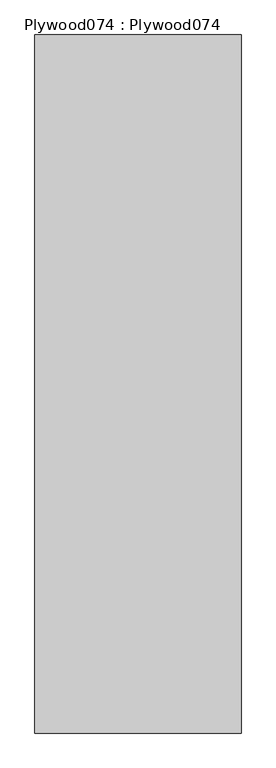
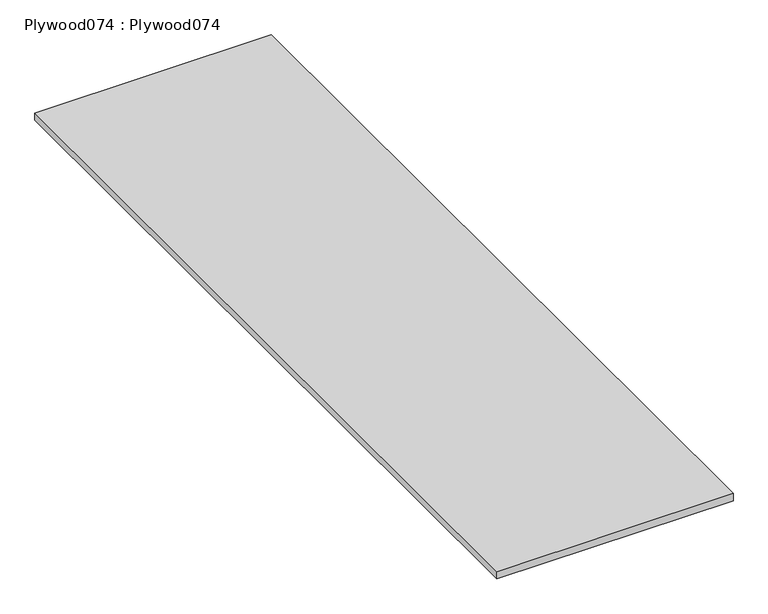
"""IFC4 building model written with IfcOpenShell, lengths in millimetres: proxy geometry, Plywood074 : Plywood074."""

from ifc_helpers import new_model, si_unit, frame, origin, place, context, project, spatial, polyline, outline, extrude, source, transform, mapped, element, save


def plywood074_plywood074_564b9597(model_context):
    return source(origin(), model_context, "Body", "SweptSolid", [
        extrude(outline(polyline([(-4404.2038825, -1052.8906574), (-4994.7538825, -1052.8906574), (-4994.7538825, 947.1093426), (-4404.2038825, 947.1093426), (-4404.2038825, -1052.8906574)])), frame((0.0, 0.0, 40112.696), z_axis=(0.0, 0.0, 1.0), x_axis=(1.0, 0.0, 0.0)), (0.0, 0.0, 1.0), 19.05),
    ])


if __name__ == "__main__":
    model = new_model("IFC4")
    model_context = context("Model", 3, world=origin())
    ifc_project = project(units=[si_unit("LENGTHUNIT", "METRE", prefix="MILLI")], contexts=[model_context])
    site = spatial("IfcSite", under=ifc_project)
    building = spatial("IfcBuilding", under=site)
    placement = place(None, origin())
    plywood074_plywood074_shape = plywood074_plywood074_564b9597(model_context)
    element("IfcBuildingElementProxy", 1, Name="Plywood074 : Plywood074", ObjectType="Plywood074 : Plywood074", at=placement, inside=building, context=model_context, shape_type="MappedRepresentation", body=[
        mapped(plywood074_plywood074_shape, transform((0.0, 0.0, 0.0), x_axis=(1.0, 0.0, 0.0), y_axis=(0.0, 1.0, 0.0), z_axis=(0.0, 0.0, 1.0))),
    ])
    save(model, "model.ifc")

# Revit data of these elements
# Type "Plywood074 : Plywood074"
#   NameOverride = "Plywood074"
# Element 1 (IfcBuildingElementProxy, "Plywood074 : Plywood074")
#   Materials on its faces: "CDX PLYWOOD -  SEE STRUCTURAL DWGS"
# Materials
#   "CDX PLYWOOD -  SEE STRUCTURAL DWGS": class "Unassigned", colour RGB 177 130 114, transparency 0, Cost = 0
